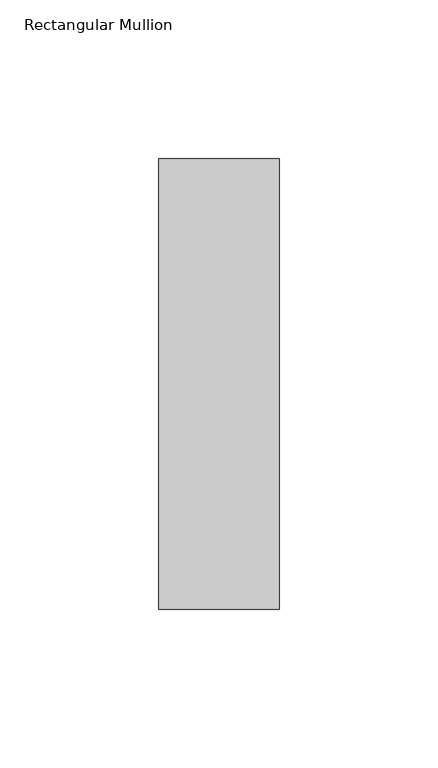
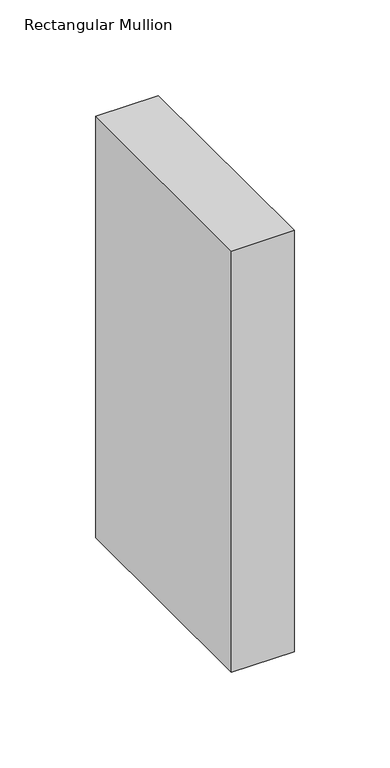
"""IFC4 building model written with IfcOpenShell, lengths in millimetres: member geometry, Rectangular Mullion : NLRS_21_CWM_hsb-regel 38x142_gen_rsf."""

from ifc_helpers import new_model, si_unit, frame, origin, place, context, project, spatial, polyline, outline, extrude, source, transform, mapped, element, save


def rectangular_mullion_985b883b(model_context):
    return source(origin(), model_context, "Body", "SweptSolid", [
        extrude(outline(polyline([(-38.0, -71.0), (-38.0, 71.0), (0.0, 71.0), (0.0, -71.0), (-38.0, -71.0)])), frame((0.0, 0.0, -269.0000003), z_axis=(0.0, 0.0, 1.0), x_axis=(1.0, 0.0, 0.0)), (0.0, 0.0, 1.0), 269.0000003),
    ])


if __name__ == "__main__":
    model = new_model("IFC4")
    model_context = context("Model", 3, world=origin())
    ifc_project = project(units=[si_unit("LENGTHUNIT", "METRE", prefix="MILLI")], contexts=[model_context])
    site = spatial("IfcSite", under=ifc_project)
    building = spatial("IfcBuilding", under=site)
    placement = place(None, origin())
    rectangular_mullion_shape = rectangular_mullion_985b883b(model_context)
    element("IfcMember", 1, ObjectType="Rectangular Mullion : NLRS_21_CWM_hsb-regel 38x142_gen_rsf", at=placement, inside=building, context=model_context, shape_type="MappedRepresentation", body=[
        mapped(rectangular_mullion_shape, transform((0.0, 0.0, 0.0), x_axis=(1.0, 0.0, 0.0), y_axis=(0.0, 1.0, 0.0), z_axis=(0.0, 0.0, 1.0))),
    ])
    save(model, "model.ifc")

# Revit data of these elements
# Type "Rectangular Mullion : NLRS_21_CWM_hsb-regel 38x142_gen_rsf"
#   Export Type to IFC As = "IfcWall"
#   Type IfcGUID = "07M7mRoiH1CR8m_RSKIwpF"
#   Assembly Code = "21.10"
#   built-in parameter 1007322 = 0.465879 (stored number, unit not read)
#   built-in parameter 1007321 = 0.062336 (stored number, unit not read)
#   built-in parameter 1007320 = 0.062336 (stored number, unit not read)
# Element 1 (IfcMember, "Rectangular Mullion : NLRS_21_CWM_hsb-regel 38x142_gen_rsf")
#   Materials on its faces: "NLRS_i2_hout naaldhout vuren_gen_rsf"
# Materials
#   "NLRS_i2_hout naaldhout vuren_gen_rsf": class "I - Hout", colour RGB 234 199 147, transparency 0, Keynote = "i2", Manufacturer = "Revit Standards Foundation", URL = "www.revitstandards.org", Description = "hout vuren", Cost = 0
